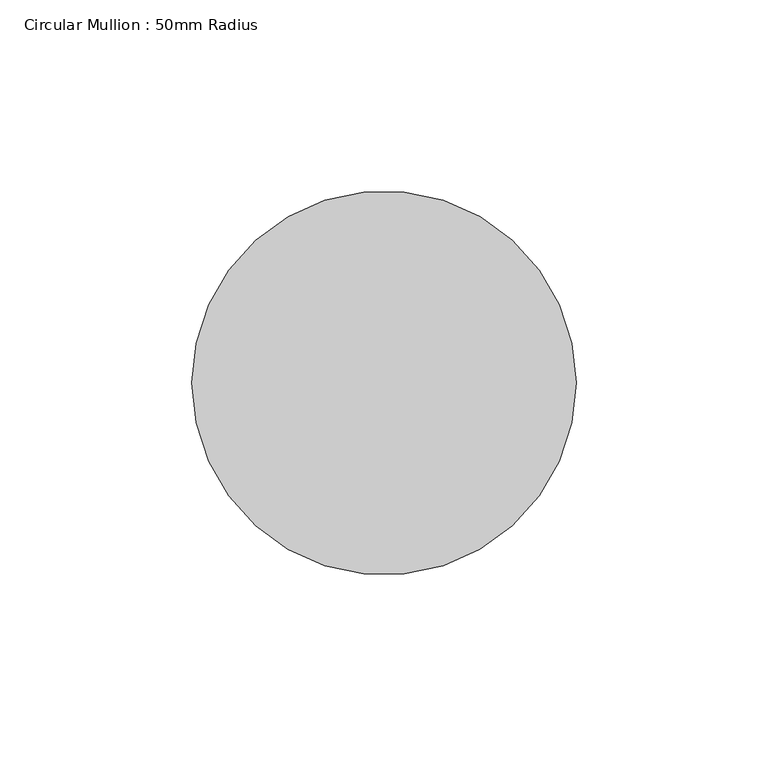
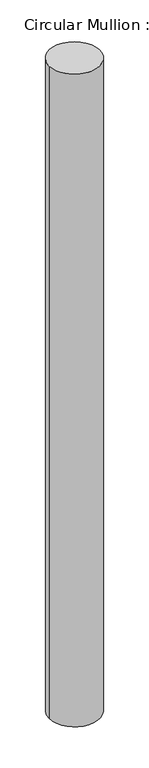
"""IFC4 building model written with IfcOpenShell, lengths in millimetres: member geometry, Circular Mullion : 50mm Radius."""

from ifc_helpers import new_model, si_unit, frame, origin, place, context, project, spatial, ellipse_curve, source, transform, mapped, element, save
from ifc_brep_helpers import plane_surface, cylinder_surface, advanced_brep


def circular_mullion_50mm_radius_b4eb7f86(model_context):
    return source(origin(), model_context, "Body", "AdvancedBrep", [
        advanced_brep(
        [(-100.0, 0.0, 0.4753902), (0.0, 0.0, 0.0), (0.0, 0.0, -1367.0207073), (-100.0, 0.0, -1367.5275642)],
        [
            (0, 1, ellipse_curve(frame((-50.0, 0.0, 0.2376951), z_axis=(-0.004753324038532295, -0.014853711216929842, -0.999878379191024), x_axis=(-0.30474659549828453, -0.9523057732188094, 0.01559573102905505)), 50.0060818, 50.0)),
            (1, 2),
            (2, 3, ellipse_curve(frame((-50.0, 0.0, -1367.2741358), z_axis=(-0.005067868536087208, -0.015836634555140575, 0.999861749300606), x_axis=(0.3047415269793715, 0.9522899345518405, 0.01662775647921587)), 50.0069135, 50.0)),
            (3, 0),
            (1, 0, ellipse_curve(frame((-50.0, 0.0, 0.2376951), z_axis=(-0.004753324038532295, -0.014853711216929842, -0.999878379191024), x_axis=(-0.30474659549828453, -0.9523057732188094, 0.01559573102905505)), 50.0060818, 50.0)),
            (3, 2, ellipse_curve(frame((-50.0, 0.0, -1367.2741358), z_axis=(-0.005067868536087208, -0.015836634555140575, 0.999861749300606), x_axis=(0.3047415269793715, 0.9522899345518405, 0.01662775647921587)), 50.0069135, 50.0)),
        ],
        [
            cylinder_surface(frame((-50.0, 0.0, 0.0), z_axis=(0.0, 0.0, 1.0), x_axis=(1.0, 0.0, 0.0)), 50.0),
            plane_surface(frame((-290.298106, 92.8980606, 0.0), z_axis=(0.004753324038532295, 0.014853711216929842, 0.999878379191024), x_axis=(0.3047465954982828, 0.9523057732188096, -0.015595731029074474))),
            plane_surface(frame((-290.298106, 92.8980606, -1367.0207073), z_axis=(0.005067868536087209, 0.015836634555140578, -0.9998617493006062), x_axis=(0.30474152697937157, 0.9522899345518407, 0.01662775647921677))),
        ],
        [
            (0, [[1, 2, 3, 4]]),
            (0, [[5, -4, 6, -2]]),
            (1, [[-1, -5]]),
            (2, [[-6, -3]]),
        ],
    ),
    ])


if __name__ == "__main__":
    model = new_model("IFC4")
    model_context = context("Model", 3, world=origin())
    ifc_project = project(units=[si_unit("LENGTHUNIT", "METRE", prefix="MILLI")], contexts=[model_context])
    site = spatial("IfcSite", under=ifc_project)
    building = spatial("IfcBuilding", under=site)
    placement = place(None, origin())
    circular_mullion_50mm_radius_shape = circular_mullion_50mm_radius_b4eb7f86(model_context)
    element("IfcMember", 1, ObjectType="Circular Mullion : 50mm Radius", at=placement, inside=building, context=model_context, shape_type="MappedRepresentation", body=[
        mapped(circular_mullion_50mm_radius_shape, transform((0.0, 0.0, 0.0), x_axis=(1.0, 0.0, 0.0), y_axis=(0.0, 1.0, 0.0), z_axis=(0.0, 0.0, 1.0))),
    ])
    save(model, "model.ifc")

# Revit data of these elements
# Type "Circular Mullion : 50mm Radius"
#   built-in parameter 1007350 = 0.164042 (stored number, unit not read)
# Element 1 (IfcMember, "Circular Mullion : 50mm Radius")
#   Materials on its faces: "Aluminium"
# Materials
#   "Aluminium": class "Metal", colour RGB 247 247 247, transparency 0, Description = "Aluminium 6061", Cost = 0
